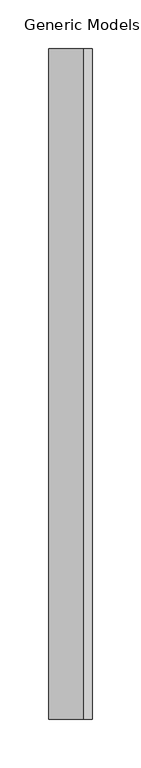
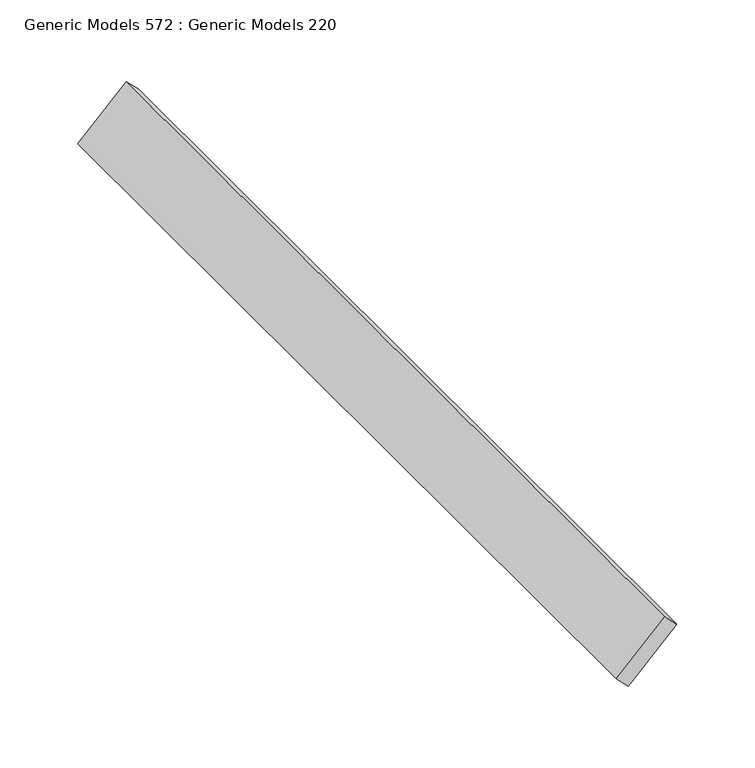
"""IFC4 building model written with IfcOpenShell, lengths in millimetres: proxy geometry, Generic Models 572 : Generic Models 220."""

from ifc_helpers import new_model, si_unit, frame, origin, place, context, project, spatial, polyline, outline, extrude, source, transform, mapped, element, save


def generic_models_572_generic_models_220_3242cf72(model_context):
    return source(origin(), model_context, "Body", "SweptSolid", [
        extrude(outline(polyline([(0.0, -12.7000001), (0.0, 0.0), (690.8142348, 0.0), (690.8142348, -12.7000001), (0.0, -12.7000001)])), frame((7841.3059863, 4539.4872686, 123985.6399101), z_axis=(0.7071067811868034, 0.0, 0.7071067811862918), x_axis=(0.0, -1.0, 0.0)), (0.0, 0.0, 1.0), 50.8),
    ])


if __name__ == "__main__":
    model = new_model("IFC4")
    model_context = context("Model", 3, world=origin())
    ifc_project = project(units=[si_unit("LENGTHUNIT", "METRE", prefix="MILLI")], contexts=[model_context])
    site = spatial("IfcSite", under=ifc_project)
    building = spatial("IfcBuilding", under=site)
    placement = place(None, origin())
    generic_models_572_generic_models_220_shape = generic_models_572_generic_models_220_3242cf72(model_context)
    element("IfcBuildingElementProxy", 1, Name="Generic Models 572 : Generic Models 220", ObjectType="Generic Models 572 : Generic Models 220", at=placement, inside=building, context=model_context, shape_type="MappedRepresentation", body=[
        mapped(generic_models_572_generic_models_220_shape, transform((0.0, 0.0, 0.0), x_axis=(1.0, 0.0, 0.0), y_axis=(0.0, 1.0, 0.0), z_axis=(0.0, 0.0, 1.0))),
    ])
    save(model, "model.ifc")

# Revit data of these elements
# Element 1 (IfcBuildingElementProxy, "Generic Models 572 : Generic Models 220")
#   Materials on its faces: "_WOOD TONE ALUMINUM EXTRUSION SLAT BY KNOTWOOD"
# Materials
#   "_WOOD TONE ALUMINUM EXTRUSION SLAT BY KNOTWOOD": class "Generic", colour RGB 177 130 114, transparency 0, Cost = 0
